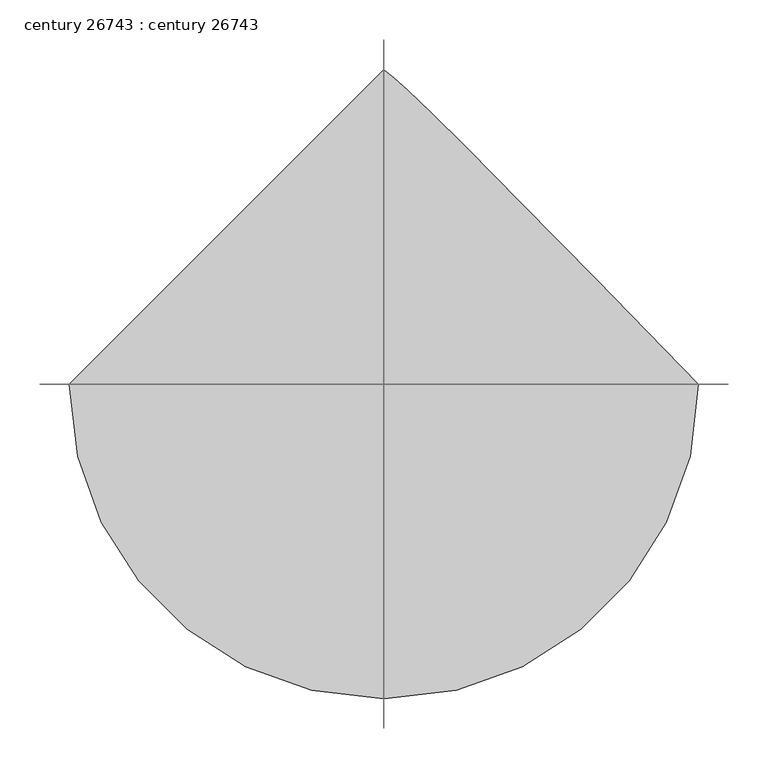
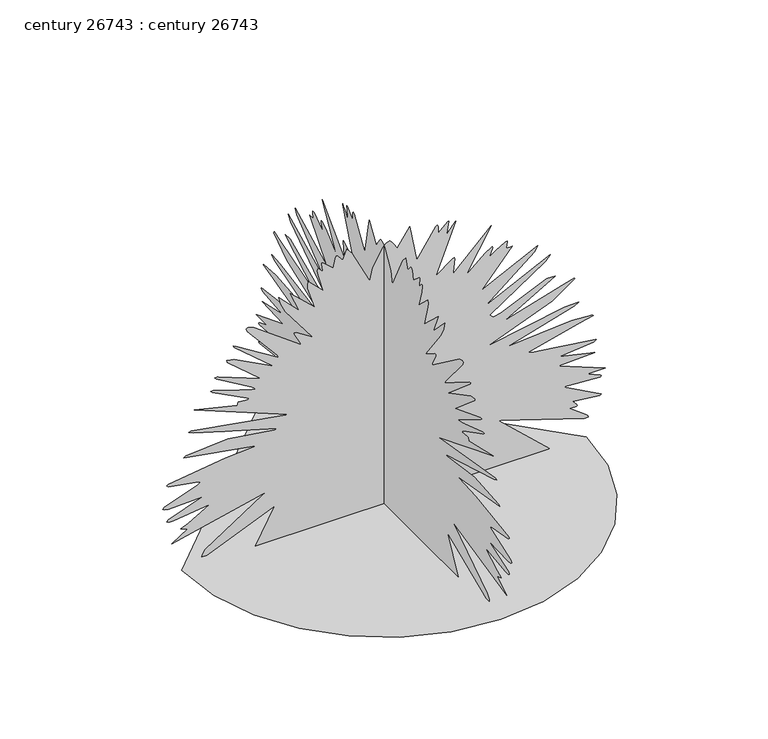
"""IFC4 building model written with IfcOpenShell, lengths in millimetres: proxy geometry, century 26743 : century 26743."""

from ifc_helpers import new_model, si_unit, origin, place, context, project, spatial, triangles, source, transform, mapped, element, save


def century_26743_century_26743_31192e91(model_context):
    return source(origin(), model_context, "Body", "Tessellation", [
        triangles([(-397.3115044, 0.0, 4.63e-05), (-386.8085844, -91.0375754, 4.63e-05), (-356.8924962, -174.6408299, 4.63e-05), (-309.9635293, -248.4147971, 4.63e-05), (-248.4147971, -309.9635293, 4.63e-05), (-174.6408299, -356.8924962, 4.63e-05), (-91.0375754, -386.8085844, 4.63e-05), (1.74e-05, -397.3115044, 4.63e-05), (91.0375754, -386.8085844, 4.63e-05), (174.6408299, -356.8924962, 4.63e-05), (248.4147971, -309.9635293, 4.63e-05), (309.9635293, -248.4147971, 4.63e-05), (356.8924962, -174.6408299, 4.63e-05), (386.8085844, -91.0375754, 4.63e-05), (397.3115044, 3.47e-05, 4.63e-05), (268.1932591, 132.4428334, 4.63e-05), (172.4726847, 229.9546048, 4.63e-05), (104.5818614, 298.3557349, 4.63e-05), (58.9551224, 343.4711497, 4.63e-05), (30.0265806, 371.1215695, 4.63e-05), (12.2302662, 387.1286593, 4.63e-05), (-5.21e-05, 397.3115044, 4.63e-05), (5.48e-05, 64.7107531, 483.8593829), (5.48e-05, 101.3189791, 540.9559705), (5.48e-05, 104.5752575, 542.8330361), (5.47e-05, 105.8282333, 541.3954059), (5.47e-05, 106.4530771, 539.3024377), (5.48e-05, 106.1718987, 525.2714991), (5.48e-05, 125.7540065, 542.1675608), (5.48e-05, 126.9272362, 542.8330361), (5.48e-05, 124.2579496, 524.65682), (5.48e-05, 123.6544436, 518.2560116), (5.48e-05, 123.7341989, 517.2882654), (5.48e-05, 126.16015, 520.6055048), (5.48e-05, 129.1273744, 524.4155193), (5.48e-05, 132.3272699, 528.3474378), (5.48e-05, 135.4524789, 532.0431061), (5.48e-05, 138.1941538, 535.1343055), (5.48e-05, 140.2449461, 537.2551789), (5.48e-05, 141.296508, 538.045138), (5.48e-05, 101.3822202, 437.4612339), (5.48e-05, 135.1415876, 462.1195398), (5.48e-05, 138.1032164, 463.0060046), (5.46e-05, 138.8316967, 460.7149017), (5.5e-05, 135.9239072, 433.9458598), (5.48e-05, 136.5068295, 431.0731427), (5.48e-05, 210.9965687, 504.766101), (5.48e-05, 160.4551951, 418.3020473), (5.44e-05, 198.6384749, 451.27627), (5.46e-05, 210.3877396, 459.3509225), (5.48e-05, 213.1421136, 459.8132126), (5.47e-05, 213.7826995, 457.8345543), (5.47e-05, 213.2487931, 455.0989655), (5.49e-05, 208.1632024, 442.6326842), (5.48e-05, 208.352435, 440.6540259), (5.46e-05, 219.9157735, 449.0715717), (5.46e-05, 238.2070626, 460.509173), (5.48e-05, 241.880403, 461.4083187), (5.48e-05, 242.4336215, 459.7675032), (5.48e-05, 240.158288, 447.6948752), (5.48e-05, 240.2837708, 447.0395737), (5.48e-05, 240.754418, 447.1106812), (5.48e-05, 242.0201111, 446.9658863), (5.48e-05, 243.8616048, 446.7144482), (5.48e-05, 246.0602351, 446.4680606), (5.48e-05, 248.3967749, 446.3334394), (5.48e-05, 250.6520333, 446.4223512), (5.48e-05, 252.6073282, 446.8388955), (5.48e-05, 192.3867853, 376.7908456), (5.48e-05, 302.5492653, 431.0731427), (5.48e-05, 296.5624941, 420.9461809), (5.48e-05, 198.7728417, 341.665228), (5.48e-05, 326.4988935, 403.9332659), (5.48e-05, 318.2667652, 392.9554112), (5.48e-05, 208.352435, 319.3132493), (5.48e-05, 214.738764, 312.9277016), (5.48e-05, 229.6693751, 315.7165938), (5.48e-05, 319.993949, 355.9552351), (5.48e-05, 336.427757, 355.8841275), (5.48e-05, 237.6894161, 297.80962), (5.48e-05, 354.2153704, 332.9123829), (5.48e-05, 374.3956429, 338.472436), (5.48e-05, 374.9087294, 336.7223974), (5.48e-05, 330.788966, 305.6429718), (5.48e-05, 203.5627746, 257.0477549), (5.48e-05, 354.9316421, 284.1952439), (5.48e-05, 382.3788403, 285.7852813), (5.48e-05, 374.1467119, 279.8975593), (5.48e-05, 243.4767991, 241.0820869), (5.48e-05, 368.8228726, 252.188731), (5.47e-05, 409.5263474, 248.5900589), (5.48e-05, 411.1163667, 247.4683977), (5.48e-05, 386.2599624, 241.4501241), (5.48e-05, 284.6880009, 215.2874042), (5.48e-05, 290.2582096, 212.731401), (5.48e-05, 337.2507082, 206.9122613), (5.48e-05, 415.7239343, 195.948868), (5.48e-05, 417.5019144, 194.7814792), (5.51e-05, 412.5921124, 191.3011866), (5.48e-05, 345.6581165, 185.2021402), (5.48e-05, 414.3091587, 169.2364723), (5.48e-05, 342.4653245, 166.0431898), (5.48e-05, 435.0660313, 129.3221935), (5.48e-05, 399.9403773, 129.3221935), (5.48e-05, 425.4470326, 118.230029), (5.48e-05, 427.0827976, 116.5495629), (5.5e-05, 424.9161784, 115.1777081), (5.55e-05, 352.3941879, 119.6112765), (5.48e-05, 427.0827976, 78.2319254), (5.48e-05, 424.5478869, 76.6512806), (5.48e-05, 371.2028509, 83.0215949), (5.48e-05, 378.6602809, 73.8036937), (5.48e-05, 379.4680078, 71.7330852), (5.48e-05, 379.1860846, 70.2489643), (5.49e-05, 377.5808046, 69.7224248), (5.48e-05, 364.8173032, 70.2489643), (5.5e-05, 396.94572, 46.9076564), (5.49e-05, 400.539832, 43.0438161), (5.48e-05, 401.5380632, 39.9142833), (5.51e-05, 393.4811786, 39.8043019), (5.48e-05, 224.3178486, 94.1975842), (5.48e-05, 326.4988935, 0.0), (5.25e-05, -253.0563924, 0.2492182), (5.48e-05, -214.738764, 70.2489643), (5.52e-05, -348.7569099, 14.888424), (5.48e-05, -358.429212, 14.369122), (5.48e-05, -357.6900856, 18.369415), (5.48e-05, -352.1731985, 27.5142681), (5.48e-05, -237.3754636, 102.1630137), (5.48e-05, -229.1077815, 105.3735736), (5.48e-05, -417.5019144, 62.266262), (5.48e-05, -385.5716323, 83.0215949), (5.48e-05, -399.1453677, 87.2423129), (5.48e-05, -399.9403773, 87.8112735), (5.48e-05, -385.228739, 93.729208), (5.48e-05, -342.4653245, 118.1462042), (5.51e-05, -414.067858, 108.9064611), (5.5e-05, -423.0289753, 109.3821952), (5.48e-05, -427.0827976, 111.7598934), (5.46e-05, -424.0398874, 115.1624746), (5.48e-05, -356.8341059, 138.9015416), (5.51e-05, -423.7858695, 136.6500893), (5.5e-05, -431.860522, 137.907389), (5.48e-05, -435.0660313, 140.4981829), (5.48e-05, -431.1315694, 144.5507516), (5.5e-05, -366.0923707, 167.5806504), (5.48e-05, -361.622004, 170.8328683), (5.47e-05, -364.7715938, 172.8602882), (5.51e-05, -423.6385674, 183.2877404), (5.48e-05, -427.0827976, 186.7985363), (5.49e-05, -424.0805099, 188.159209), (5.49e-05, -311.5713527, 203.8116875), (5.49e-05, -256.2933678, 207.4789418), (5.48e-05, -253.0563924, 209.1505149), (5.48e-05, -393.5548296, 233.0991258), (5.46e-05, -389.6000565, 235.80601), (5.48e-05, -307.626717, 241.9065642), (5.51e-05, -214.7303706, 227.9886456), (5.48e-05, -209.948831, 229.9060976), (5.49e-05, -316.3643014, 260.8094802), (5.5e-05, -375.017916, 278.0992497), (5.48e-05, -383.9739464, 282.5925074), (5.47e-05, -378.9168423, 283.5526232), (5.48e-05, -186.0004563, 250.6614259), (5.48e-05, -372.7979934, 325.7013405), (5.48e-05, -288.1805021, 304.9444679), (5.48e-05, -286.5853778, 311.330052), (5.49e-05, -269.0365398, 309.9889275), (5.49e-05, -266.8318233, 310.4054718), (5.48e-05, -265.8285234, 311.330052), (5.51e-05, -269.4886561, 314.5837778), (5.5e-05, -337.4081841, 349.4630078), (5.48e-05, -340.8676749, 352.8412173), (5.47e-05, -335.5743207, 352.5516638), (5.53e-05, -271.7060716, 331.7160533), (5.52e-05, -258.9603743, 327.9466976), (5.48e-05, -253.0563924, 327.2964466), (5.47e-05, -256.1943004, 330.9845209), (5.49e-05, -329.3817844, 374.403237), (5.48e-05, -332.8844413, 378.3859517), (5.47e-05, -327.5276098, 378.3301048), (5.48e-05, -241.880403, 344.85802), (5.49e-05, -308.2058241, 401.9647814), (5.48e-05, -308.9373565, 405.528372), (5.48e-05, -294.7489238, 403.1128581), (5.48e-05, -217.9317922, 362.4221005), (5.49e-05, -294.4847684, 427.674622), (5.48e-05, -296.1637176, 431.0731427), (5.41e-05, -290.0245392, 428.8582706), (5.42e-05, -241.5682491, 398.2563595), (5.48e-05, -206.7558028, 376.7908456), (5.48e-05, -209.5086508, 382.4067819), (5.5e-05, -268.4244042, 452.4624621), (5.48e-05, -270.6189468, 458.215563), (5.47e-05, -268.9298603, 459.1502807), (5.46e-05, -266.5473385, 459.2798149), (5.48e-05, -256.0139699, 455.7949259), (5.48e-05, -163.6484776, 387.9668349), (5.5e-05, -163.5410351, 390.7938426), (5.49e-05, -176.684001, 414.5987123), (5.48e-05, -176.420863, 416.7043613), (5.45e-05, -172.2849781, 416.6180294), (5.48e-05, -139.6998668, 395.9500686), (5.48e-05, -193.7675149, 467.5119432), (5.48e-05, -203.1330043, 485.9548582), (5.48e-05, -206.7558028, 501.3218345), (5.48e-05, -166.8415059, 459.8132126), (5.48e-05, -184.4038241, 501.3218345), (5.48e-05, -136.5068295, 456.6178771), (5.48e-05, -149.7757779, 500.0289991), (5.48e-05, -150.1494106, 507.4153215), (5.48e-05, -149.2792058, 514.0955097), (5.48e-05, -118.9445294, 485.3579833), (5.43e-05, -128.2922237, 517.4533716), (5.44e-05, -130.742056, 529.9577682), (5.48e-05, -130.1205187, 533.2546964), (5.47e-05, -128.9290035, 533.6280747), (5.47e-05, -127.6127775, 532.9753166), (5.49e-05, -121.6623231, 526.7091293), (5.49e-05, -120.1429028, 525.8836347), (5.49e-05, -119.9783053, 528.2077297), (5.48e-05, -122.302146, 540.4911369), (5.48e-05, -122.1375576, 542.8330361), (5.46e-05, -119.638455, 542.3428044), (5.48e-05, -102.0654815, 526.4195758), (5.48e-05, -99.7855789, 525.2714991), (5.46e-05, -95.8008294, 543.3384922), (5.47e-05, -94.7246324, 545.9445105), (5.48e-05, -93.3992681, 547.6234777), (5.47e-05, -91.253478, 547.0443343), (5.48e-05, -80.6268828, 534.8498025), (5.48e-05, -73.7094589, 554.268094), (5.48e-05, -73.292642, 554.7583257), (5.48e-05, -63.1898021, 543.4502586), (5.48e-05, -27.9399734, 472.5843081), (5.44e-05, -22.4150971, 498.3830604), (5.38e-05, -2.3979102, 533.6128504), (5.41e-05, 4.5262249, 540.3336611), (5.48e-05, 10.3776937, 542.8330361), (5.48e-05, 12.3454038, 541.6722422), (5.48e-05, 14.9915223, 538.702983), (5.48e-05, 17.9716002, 534.6491607), (5.48e-05, 20.9412636, 530.2371843), (5.48e-05, 23.5559886, 526.1858691), (5.48e-05, 25.4716034, 523.2267838), (5.48e-05, 26.3433298, 522.078707), (5.48e-05, 50.291952, 558.7994671), (64.7107531, 5.24e-05, 483.8593829), (101.3189791, 4.9e-05, 540.9559705), (104.5752575, 4.89e-05, 542.8330361), (105.8282333, 4.9e-05, 541.3954059), (106.4530771, 4.92e-05, 539.3024377), (106.1718987, 4.99e-05, 525.2714991), (125.7540065, 4.89e-05, 542.1675608), (126.9272362, 4.89e-05, 542.8330361), (124.2579496, 4.99e-05, 524.65682), (123.6544436, 5.03e-05, 518.2560116), (123.7341989, 5.04e-05, 517.2882654), (126.16015, 5.02e-05, 520.6055048), (129.1273744, 4.99e-05, 524.4155193), (132.3272699, 4.97e-05, 528.3474378), (135.4524789, 4.95e-05, 532.0431061), (138.1941538, 4.93e-05, 535.1343055), (140.2449461, 4.92e-05, 537.2551789), (141.296508, 4.91e-05, 538.045138), (101.3822202, 5.51e-05, 437.4612339), (135.1415876, 5.37e-05, 462.1195398), (138.1032164, 5.36e-05, 463.0060046), (138.8316967, 5.4e-05, 460.7149017), (135.9239072, 5.52e-05, 433.9458598), (136.5068295, 5.55e-05, 431.0731427), (210.9965687, 5.11e-05, 504.766101), (160.4551951, 5.63e-05, 418.3020473), (198.6384749, 5.47e-05, 451.27627), (210.3877396, 5.41e-05, 459.3509225), (213.1421136, 5.38e-05, 459.8132126), (213.7826995, 5.4e-05, 457.8345543), (213.2487931, 5.42e-05, 455.0989655), (208.1632024, 5.47e-05, 442.6326842), (208.352435, 5.49e-05, 440.6540259), (219.9157735, 5.47e-05, 449.0715717), (238.2070626, 5.4e-05, 460.509173), (241.880403, 5.37e-05, 461.4083187), (242.4336215, 5.39e-05, 459.7675032), (240.158288, 5.45e-05, 447.6948752), (240.2837708, 5.46e-05, 447.0395737), (240.754418, 5.46e-05, 447.1106812), (242.0201111, 5.46e-05, 446.9658863), (243.8616048, 5.46e-05, 446.7144482), (246.0602351, 5.46e-05, 446.4680606), (248.3967749, 5.46e-05, 446.3334394), (250.6520333, 5.46e-05, 446.4223512), (252.6073282, 5.46e-05, 446.8388955), (192.3867853, 5.87e-05, 376.7908456), (302.5492653, 5.55e-05, 431.0731427), (296.5624941, 5.61e-05, 420.9461809), (198.7728417, 6.08e-05, 341.665228), (326.4988935, 5.71e-05, 403.9332659), (318.2667652, 5.78e-05, 392.9554112), (208.352435, 6.22e-05, 319.3132493), (214.738764, 6.26e-05, 312.9277016), (229.6693751, 6.24e-05, 315.7165938), (319.993949, 6e-05, 355.9552351), (336.427757, 6e-05, 355.8841275), (237.6894161, 6.35e-05, 297.80962), (354.2153704, 6.14e-05, 332.9123829), (374.3956429, 6.1e-05, 338.472436), (374.9087294, 6.11e-05, 336.7223974), (330.788966, 6.3e-05, 305.6429718), (203.5627746, 6.59e-05, 257.0477549), (354.9316421, 6.43e-05, 284.1952439), (382.3788403, 6.42e-05, 285.7852813), (374.1467119, 6.45e-05, 279.8975593), (243.4767991, 6.68e-05, 241.0820869), (368.8228726, 6.62e-05, 252.188731), (409.5263474, 6.65e-05, 248.5900589), (411.1163667, 6.65e-05, 247.4683977), (386.2599624, 6.69e-05, 241.4501241), (284.6880009, 6.84e-05, 215.2874042), (290.2582096, 6.85e-05, 212.731401), (337.2507082, 6.89e-05, 206.9122613), (415.7239343, 6.96e-05, 195.948868), (417.5019144, 6.96e-05, 194.7814792), (412.5921124, 6.95e-05, 191.3011866), (345.6581165, 7.02e-05, 185.2021402), (414.3091587, 7.11e-05, 169.2364723), (342.4653245, 7.13e-05, 166.0431898), (435.0660313, 7.35e-05, 129.3221935), (399.9403773, 7.35e-05, 129.3221935), (425.4470326, 7.41e-05, 118.230029), (427.0827976, 7.43e-05, 116.5495629), (424.9161784, 7.42e-05, 115.1777081), (352.3941879, 7.34e-05, 119.6112765), (427.0827976, 7.65e-05, 78.2319254), (424.5478869, 7.66e-05, 76.6512806), (371.2028509, 7.63e-05, 83.0215949), (378.6602809, 7.69e-05, 73.8036937), (379.4680078, 7.7e-05, 71.7330852), (379.1860846, 7.7e-05, 70.2489643), (377.5808046, 7.7e-05, 69.7224248), (364.8173032, 7.7e-05, 70.2489643), (396.94572, 7.82e-05, 46.9076564), (400.539832, 7.85e-05, 43.0438161), (401.5380632, 7.88e-05, 39.9142833), (393.4811786, 7.86e-05, 39.8043019), (224.3178486, 7.56e-05, 94.1975842), (326.4988935, 8.12e-05, 1.09e-05), (-253.0563924, 8.35e-05, 0.2492291), (-214.738764, 7.7e-05, 70.2489643), (-348.7569099, 7.99e-05, 14.888449), (-358.429212, 8.03e-05, 14.369147), (-357.6900856, 8.01e-05, 18.369415), (-352.1731985, 7.96e-05, 27.5142681), (-237.3754636, 7.51e-05, 102.1630137), (-229.1077815, 7.49e-05, 105.3735736), (-417.5019144, 7.75e-05, 62.266262), (-385.5716323, 7.63e-05, 83.0215949), (-399.1453677, 7.6e-05, 87.2423129), (-399.9403773, 7.6e-05, 87.8112735), (-385.228739, 7.56e-05, 93.729208), (-342.4653245, 7.42e-05, 118.1462042), (-414.067858, 7.44e-05, 108.9064611), (-423.0289753, 7.45e-05, 109.3821952), (-427.0827976, 7.45e-05, 111.7598934), (-424.0398874, 7.45e-05, 115.1624746), (-356.8341059, 7.29e-05, 138.9015416), (-423.7858695, 7.28e-05, 136.6500893), (-431.860522, 7.28e-05, 137.907389), (-435.0660313, 7.28e-05, 140.4981829), (-431.1315694, 7.26e-05, 144.5507516), (-366.0923707, 7.1e-05, 167.5806504), (-361.622004, 7.1e-05, 170.8328683), (-364.7715938, 7.1e-05, 172.8602882), (-423.6385674, 7e-05, 183.2877404), (-427.0827976, 7.01e-05, 186.7985363), (-424.0805099, 6.99e-05, 188.159209), (-311.5713527, 6.9e-05, 203.8116875), (-256.2933678, 6.88e-05, 207.4789418), (-253.0563924, 6.87e-05, 209.1505149), (-393.5548296, 6.73e-05, 233.0991258), (-389.6000565, 6.74e-05, 235.80601), (-307.626717, 6.68e-05, 241.9065642), (-214.7303706, 6.74e-05, 227.9886456), (-209.948831, 6.75e-05, 229.9060976), (-316.3643014, 6.56e-05, 260.8094802), (-375.017916, 6.45e-05, 278.0992497), (-383.9739464, 6.44e-05, 282.5925074), (-378.9168423, 6.45e-05, 283.5526232), (-186.0004563, 6.63e-05, 250.6614259), (-372.7979934, 6.18e-05, 325.7013405), (-288.1805021, 6.3e-05, 304.9444679), (-286.5853778, 6.26e-05, 311.330052), (-269.0365398, 6.26e-05, 309.9889275), (-266.8318233, 6.26e-05, 310.4054718), (-265.8285234, 6.26e-05, 311.330052), (-269.4886561, 6.21e-05, 314.5837778), (-337.4081841, 6.02e-05, 349.4630078), (-340.8676749, 6.02e-05, 352.8412173), (-335.5743207, 6.03e-05, 352.5516638), (-271.7060716, 6.1e-05, 331.7160533), (-258.9603743, 6.13e-05, 327.9466976), (-253.0563924, 6.17e-05, 327.2964466), (-256.1943004, 6.16e-05, 330.9845209), (-329.3817844, 5.88e-05, 374.403237), (-332.8844413, 5.87e-05, 378.3859517), (-327.5276098, 5.88e-05, 378.3301048), (-241.880403, 6.07e-05, 344.85802), (-308.2058241, 5.71e-05, 401.9647814), (-308.9373565, 5.7e-05, 405.528372), (-294.7489238, 5.72e-05, 403.1128581), (-217.9317922, 5.96e-05, 362.4221005), (-294.4847684, 5.57e-05, 427.674622), (-296.1637176, 5.55e-05, 431.0731427), (-290.0245392, 5.63e-05, 428.8582706), (-241.5682491, 5.81e-05, 398.2563595), (-206.7558028, 5.87e-05, 376.7908456), (-209.5086508, 5.84e-05, 382.4067819), (-268.4244042, 5.41e-05, 452.4624621), (-270.6189468, 5.39e-05, 458.215563), (-268.9298603, 5.4e-05, 459.1502807), (-266.5473385, 5.4e-05, 459.2798149), (-256.0139699, 5.41e-05, 455.7949259), (-163.6484776, 5.81e-05, 387.9668349), (-163.5410351, 5.77e-05, 390.7938426), (-176.684001, 5.64e-05, 414.5987123), (-176.420863, 5.64e-05, 416.7043613), (-172.2849781, 5.67e-05, 416.6180294), (-139.6998668, 5.76e-05, 395.9500686), (-193.7675149, 5.33e-05, 467.5119432), (-203.1330043, 5.22e-05, 485.9548582), (-206.7558028, 5.13e-05, 501.3218345), (-166.8415059, 5.38e-05, 459.8132126), (-184.4038241, 5.13e-05, 501.3218345), (-136.5068295, 5.4e-05, 456.6178771), (-149.7757779, 5.14e-05, 500.0289991), (-150.1494106, 5.1e-05, 507.4153215), (-149.2792058, 5.06e-05, 514.0955097), (-118.9445294, 5.23e-05, 485.3579833), (-128.2922237, 5.09e-05, 517.4533716), (-130.742056, 5e-05, 529.9577682), (-130.1205187, 4.94e-05, 533.2546964), (-128.9290035, 4.95e-05, 533.6280747), (-127.6127775, 4.95e-05, 532.9753166), (-121.6623231, 4.97e-05, 526.7091293), (-120.1429028, 4.98e-05, 525.8836347), (-119.9783053, 4.96e-05, 528.2077297), (-122.302146, 4.9e-05, 540.4911369), (-122.1375576, 4.89e-05, 542.8330361), (-119.638455, 4.91e-05, 542.3428044), (-102.0654815, 4.99e-05, 526.4195758), (-99.7855789, 4.99e-05, 525.2714991), (-95.8008294, 4.9e-05, 543.3384922), (-94.7246324, 4.88e-05, 545.9445105), (-93.3992681, 4.86e-05, 547.6234777), (-91.253478, 4.87e-05, 547.0443343), (-80.6268828, 4.93e-05, 534.8498025), (-73.7094589, 4.82e-05, 554.268094), (-73.292642, 4.81e-05, 554.7583257), (-63.1898021, 4.88e-05, 543.4502586), (-27.9399734, 5.3e-05, 472.5843081), (-22.4150971, 5.19e-05, 498.3830604), (-2.3979102, 5.04e-05, 533.6128504), (4.5262249, 4.97e-05, 540.3336611), (10.3776937, 4.89e-05, 542.8330361), (12.3454038, 4.89e-05, 541.6722422), (14.9915223, 4.91e-05, 538.702983), (17.9716002, 4.93e-05, 534.6491607), (20.9412636, 4.96e-05, 530.2371843), (23.5559886, 4.98e-05, 526.1858691), (25.4716034, 5e-05, 523.2267838), (26.3433298, 5.01e-05, 522.078707), (50.291952, 4.79e-05, 558.7994671)], [[21, 22, 1], [20, 21, 1], [19, 20, 1], [18, 19, 1], [17, 18, 1], [17, 1, 2], [17, 2, 3], [17, 3, 4], [16, 17, 4], [16, 4, 5], [16, 5, 6], [16, 6, 7], [16, 7, 8], [16, 8, 9], [16, 9, 10], [16, 10, 11], [16, 11, 12], [15, 16, 12], [14, 15, 12], [13, 14, 12], [164, 165, 166], [46, 47, 48], [100, 101, 102], [130, 131, 132], [102, 103, 104], [207, 208, 209], [72, 73, 74], [72, 74, 75], [205, 206, 207], [204, 205, 207], [78, 79, 80], [39, 40, 41], [38, 39, 41], [37, 38, 41], [36, 37, 41], [35, 36, 41], [34, 35, 41], [33, 34, 41], [86, 87, 88], [86, 88, 89], [69, 70, 71], [69, 71, 72], [67, 68, 69], [161, 162, 163], [172, 173, 174], [121, 122, 123], [187, 188, 189], [246, 247, 23], [154, 155, 156], [154, 156, 157], [77, 78, 80], [66, 67, 69], [179, 180, 181], [91, 92, 93], [90, 91, 93], [121, 123, 124], [29, 30, 31], [133, 134, 135], [132, 133, 135], [211, 212, 213], [210, 211, 213], [65, 66, 69], [85, 86, 89], [64, 65, 69], [187, 189, 190], [186, 187, 190], [108, 109, 110], [108, 110, 111], [63, 64, 69], [62, 63, 69], [61, 62, 69], [97, 98, 99], [183, 184, 185], [149, 150, 151], [118, 119, 120], [117, 118, 120], [125, 126, 127], [105, 106, 107], [138, 139, 140], [160, 161, 163], [160, 163, 164], [159, 160, 164], [232, 233, 234], [231, 232, 234], [222, 223, 224], [186, 190, 191], [143, 144, 145], [96, 97, 99], [172, 174, 175], [171, 172, 175], [171, 175, 176], [81, 82, 83], [81, 83, 84], [42, 43, 44], [96, 99, 100], [182, 183, 185], [142, 143, 145], [141, 142, 145], [170, 171, 176], [203, 204, 207], [203, 207, 209], [141, 145, 146], [57, 58, 59], [89, 90, 93], [89, 93, 94], [81, 84, 85], [80, 81, 85], [200, 201, 202], [148, 149, 151], [148, 151, 152], [178, 179, 181], [178, 181, 182], [177, 178, 182], [193, 194, 195], [193, 195, 196], [166, 167, 168], [164, 166, 168], [164, 168, 169], [164, 169, 170], [50, 51, 52], [116, 117, 120], [24, 25, 26], [24, 26, 27], [137, 138, 140], [136, 137, 140], [136, 140, 141], [50, 52, 53], [49, 50, 53], [49, 53, 54], [49, 54, 55], [76, 77, 80], [76, 80, 85], [125, 127, 128], [124, 125, 128], [124, 128, 129], [124, 129, 130], [199, 200, 202], [182, 185, 186], [147, 148, 152], [164, 170, 176], [164, 176, 177], [104, 105, 107], [104, 107, 108], [102, 104, 108], [193, 196, 197], [192, 193, 197], [192, 197, 198], [191, 192, 198], [164, 177, 182], [164, 182, 186], [141, 146, 147], [130, 132, 135], [130, 135, 136], [121, 124, 130], [221, 222, 224], [28, 29, 31], [28, 31, 32], [41, 42, 44], [41, 44, 45], [23, 24, 27], [23, 27, 28], [209, 210, 213], [199, 202, 203], [198, 199, 203], [221, 224, 225], [220, 221, 225], [154, 157, 158], [228, 229, 230], [56, 57, 59], [56, 59, 60], [116, 120, 121], [28, 32, 33], [28, 33, 41], [23, 28, 41], [215, 216, 217], [215, 217, 218], [214, 215, 218], [214, 218, 219], [214, 219, 220], [113, 114, 115], [112, 113, 115], [111, 112, 115], [41, 45, 46], [111, 115, 116], [214, 220, 225], [214, 225, 226], [96, 100, 102], [56, 60, 61], [56, 61, 69], [55, 56, 69], [49, 55, 69], [48, 49, 69], [111, 116, 121], [108, 111, 121], [102, 108, 121], [96, 102, 121], [95, 96, 121], [94, 95, 121], [89, 94, 121], [89, 121, 130], [85, 89, 130], [76, 85, 130], [75, 76, 130], [72, 75, 130], [69, 72, 130], [48, 69, 130], [46, 48, 130], [41, 46, 130], [23, 41, 130], [246, 23, 130], [245, 246, 130], [244, 245, 130], [243, 244, 130], [242, 243, 130], [241, 242, 130], [240, 241, 130], [227, 228, 230], [227, 230, 231], [226, 227, 231], [141, 147, 152], [136, 141, 152], [130, 136, 152], [130, 152, 153], [130, 153, 154], [130, 154, 158], [130, 158, 159], [164, 186, 191], [164, 191, 198], [164, 198, 203], [238, 239, 240], [231, 234, 235], [226, 231, 235], [214, 226, 235], [213, 214, 235], [209, 213, 235], [203, 209, 235], [130, 159, 164], [164, 203, 235], [237, 238, 240], [236, 237, 240], [235, 236, 240], [235, 240, 130], [164, 235, 130], [389, 390, 391], [271, 272, 273], [325, 326, 327], [355, 356, 357], [327, 328, 329], [432, 433, 434], [297, 298, 299], [297, 299, 300], [430, 431, 432], [429, 430, 432], [303, 304, 305], [264, 265, 266], [263, 264, 266], [262, 263, 266], [261, 262, 266], [260, 261, 266], [259, 260, 266], [258, 259, 266], [311, 312, 313], [311, 313, 314], [294, 295, 296], [294, 296, 297], [292, 293, 294], [386, 387, 388], [397, 398, 399], [346, 347, 348], [412, 413, 414], [471, 472, 248], [379, 380, 381], [379, 381, 382], [302, 303, 305], [291, 292, 294], [404, 405, 406], [316, 317, 318], [315, 316, 318], [346, 348, 349], [254, 255, 256], [358, 359, 360], [357, 358, 360], [436, 437, 438], [435, 436, 438], [290, 291, 294], [310, 311, 314], [289, 290, 294], [412, 414, 415], [411, 412, 415], [333, 334, 335], [333, 335, 336], [288, 289, 294], [287, 288, 294], [286, 287, 294], [322, 323, 324], [408, 409, 410], [374, 375, 376], [343, 344, 345], [342, 343, 345], [350, 351, 352], [330, 331, 332], [363, 364, 365], [385, 386, 388], [385, 388, 389], [384, 385, 389], [457, 458, 459], [456, 457, 459], [447, 448, 449], [411, 415, 416], [368, 369, 370], [321, 322, 324], [397, 399, 400], [396, 397, 400], [396, 400, 401], [306, 307, 308], [306, 308, 309], [267, 268, 269], [321, 324, 325], [407, 408, 410], [367, 368, 370], [366, 367, 370], [395, 396, 401], [428, 429, 432], [428, 432, 434], [366, 370, 371], [282, 283, 284], [314, 315, 318], [314, 318, 319], [306, 309, 310], [305, 306, 310], [425, 426, 427], [373, 374, 376], [373, 376, 377], [403, 404, 406], [403, 406, 407], [402, 403, 407], [418, 419, 420], [418, 420, 421], [391, 392, 393], [389, 391, 393], [389, 393, 394], [389, 394, 395], [275, 276, 277], [341, 342, 345], [249, 250, 251], [249, 251, 252], [362, 363, 365], [361, 362, 365], [361, 365, 366], [275, 277, 278], [274, 275, 278], [274, 278, 279], [274, 279, 280], [301, 302, 305], [301, 305, 310], [350, 352, 353], [349, 350, 353], [349, 353, 354], [349, 354, 355], [424, 425, 427], [407, 410, 411], [372, 373, 377], [389, 395, 401], [389, 401, 402], [329, 330, 332], [329, 332, 333], [327, 329, 333], [418, 421, 422], [417, 418, 422], [417, 422, 423], [416, 417, 423], [389, 402, 407], [389, 407, 411], [366, 371, 372], [355, 357, 360], [355, 360, 361], [346, 349, 355], [446, 447, 449], [253, 254, 256], [253, 256, 257], [266, 267, 269], [266, 269, 270], [248, 249, 252], [248, 252, 253], [434, 435, 438], [424, 427, 428], [423, 424, 428], [446, 449, 450], [445, 446, 450], [379, 382, 383], [453, 454, 455], [281, 282, 284], [281, 284, 285], [341, 345, 346], [253, 257, 258], [253, 258, 266], [248, 253, 266], [440, 441, 442], [440, 442, 443], [439, 440, 443], [439, 443, 444], [439, 444, 445], [338, 339, 340], [337, 338, 340], [336, 337, 340], [266, 270, 271], [336, 340, 341], [439, 445, 450], [439, 450, 451], [321, 325, 327], [281, 285, 286], [281, 286, 294], [280, 281, 294], [274, 280, 294], [273, 274, 294], [336, 341, 346], [333, 336, 346], [327, 333, 346], [321, 327, 346], [320, 321, 346], [319, 320, 346], [314, 319, 346], [314, 346, 355], [310, 314, 355], [301, 310, 355], [300, 301, 355], [297, 300, 355], [294, 297, 355], [273, 294, 355], [271, 273, 355], [266, 271, 355], [248, 266, 355], [471, 248, 355], [470, 471, 355], [469, 470, 355], [468, 469, 355], [467, 468, 355], [466, 467, 355], [465, 466, 355], [452, 453, 455], [452, 455, 456], [451, 452, 456], [366, 372, 377], [361, 366, 377], [355, 361, 377], [355, 377, 378], [355, 378, 379], [355, 379, 383], [355, 383, 384], [389, 411, 416], [389, 416, 423], [389, 423, 428], [463, 464, 465], [456, 459, 460], [451, 456, 460], [439, 451, 460], [438, 439, 460], [434, 438, 460], [428, 434, 460], [355, 384, 389], [389, 428, 460], [462, 463, 465], [461, 462, 465], [460, 461, 465], [460, 465, 355], [389, 460, 355]], closed=False),
    ])


if __name__ == "__main__":
    model = new_model("IFC4")
    model_context = context("Model", 3, world=origin())
    ifc_project = project(units=[si_unit("LENGTHUNIT", "METRE", prefix="MILLI")], contexts=[model_context])
    site = spatial("IfcSite", under=ifc_project)
    building = spatial("IfcBuilding", under=site)
    placement = place(None, origin())
    century_26743_century_26743_shape = century_26743_century_26743_31192e91(model_context)
    element("IfcBuildingElementProxy", 1, Name="century 26743 : century 26743", ObjectType="century 26743 : century 26743", at=placement, inside=building, context=model_context, shape_type="MappedRepresentation", body=[
        mapped(century_26743_century_26743_shape, transform((0.0, 0.0, 0.0), x_axis=(1.0, 0.0, 0.0), y_axis=(0.0, 1.0, 0.0), z_axis=(0.0, 0.0, 1.0))),
    ])
    save(model, "model.ifc")

# Revit data of these elements
# Type "century 26743 : century 26743"
#   built-in parameter 1005195 = "RPC-16-FXAD-JSXX-UCRP-S000-ST1L-LVER-AU"
#   Height = 0
